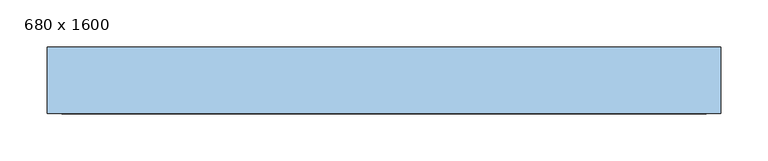
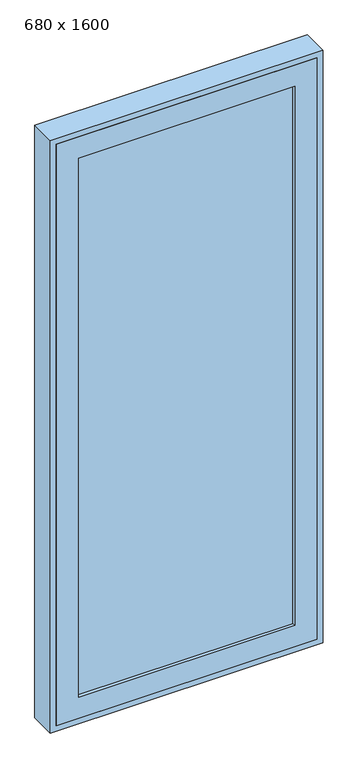
"""IFC4 building model written with IfcOpenShell, lengths in millimetres: window geometry, Aluprof_MB-79N-SI_E_Alu_Window-1sash-FIX_ENG_R-00206 : 680 x 1600."""

from ifc_helpers import new_model, si_unit, frame, origin, place, context, project, spatial, polyline, outline, extrude, faceted_brep, source, transform, mapped, element, save


def window_680_x_1600_1ad14e31(model_context):
    return source(origin(), model_context, "Body", "SolidModel", [
        faceted_brep([(-284.5, -58.5, 2315.5), (-284.5, -58.5, 826.5), (-284.5, -45.0, 826.5), (-284.5, -45.0, 2315.5), (-340.0, -45.0, 2371.0), (-340.0, -45.0, 771.0), (-340.0, -115.0, 771.0), (-340.0, -115.0, 2371.0), (284.5, -58.5, 826.5), (284.5, -45.0, 826.5), (340.0, -45.0, 771.0), (340.0, -115.0, 771.0), (284.5, -58.5, 2315.5), (284.5, -45.0, 2315.5), (340.0, -45.0, 2371.0), (340.0, -115.0, 2371.0), (-300.5, -58.5, 2331.5), (-300.5, -58.5, 810.5), (300.5, -58.5, 810.5), (300.5, -58.5, 2331.5), (-300.5, -106.5, 2331.5), (-300.5, -106.5, 810.5), (300.5, -106.5, 810.5), (300.5, -106.5, 2331.5), (-281.5, -106.5, 2312.5), (-281.5, -106.5, 829.5), (281.5, -106.5, 829.5), (281.5, -106.5, 2312.5), (-281.5, -115.0, 2312.5), (-281.5, -115.0, 829.5), (281.5, -115.0, 829.5), (281.5, -115.0, 2312.5)], [[[0, 1, 2, 3]], [[4, 5, 6, 7]], [[1, 8, 9, 2]], [[5, 10, 11, 6]], [[8, 12, 13, 9]], [[10, 14, 15, 11]], [[16, 17, 18, 19], [1, 0, 12, 8]], [[12, 0, 3, 13]], [[5, 4, 14, 10], [3, 2, 9, 13]], [[14, 4, 7, 15]], [[20, 21, 17, 16]], [[21, 22, 18, 17]], [[22, 23, 19, 18]], [[21, 20, 23, 22], [24, 25, 26, 27]], [[23, 20, 16, 19]], [[28, 29, 25, 24]], [[29, 30, 26, 25]], [[30, 31, 27, 26]], [[7, 6, 11, 15], [29, 28, 31, 30]], [[31, 28, 24, 27]]]),
        extrude(outline(polyline([(300.5, -58.5), (300.5, -106.5), (-300.5, -106.5), (-300.5, -58.5), (300.5, -58.5)])), frame((0.0, 0.0, 810.5), z_axis=(0.0, 0.0, 1.0), x_axis=(1.0, 0.0, 0.0)), (0.0, 0.0, 1.0), 1521.0),
        extrude(outline(polyline([(2386.0, -355.0), (756.0, -355.0), (756.0, 355.0), (2386.0, 355.0), (2386.0, -355.0)]), holes=[polyline([(771.0, -340.0), (2371.0, -340.0), (2371.0, 340.0), (771.0, 340.0), (771.0, -340.0)])]), frame((0.0, -115.0, 0.0), z_axis=(0.0, 1.0, 0.0), x_axis=(0.0, 0.0, 1.0)), (0.0, 0.0, 1.0), 70.0),
    ])


if __name__ == "__main__":
    model = new_model("IFC4")
    model_context = context("Model", 3, world=origin())
    ifc_project = project(units=[si_unit("LENGTHUNIT", "METRE", prefix="MILLI")], contexts=[model_context])
    site = spatial("IfcSite", under=ifc_project)
    building = spatial("IfcBuilding", under=site)
    placement = place(None, origin())
    window_680_x_1600_shape = window_680_x_1600_1ad14e31(model_context)
    element("IfcWindow", 1, ObjectType="Aluprof_MB-79N-SI_E_Alu_Window-1sash-FIX_ENG_R-00206 : 680 x 1600", at=placement, inside=building, context=model_context, shape_type="MappedRepresentation", body=[
        mapped(window_680_x_1600_shape, transform((0.0, 0.0, 0.0), x_axis=(1.0, 0.0, 0.0), y_axis=(0.0, 1.0, 0.0), z_axis=(0.0, 0.0, 1.0))),
    ])
    save(model, "model.ifc")

# Revit data of these elements
# Type "Aluprof_MB-79N-SI_E_Alu_Window-1sash-FIX_ENG_R-00206 : 680 x 1600"
#   Type Mark = "50"
#   Water resistance = "Class E1950, EN 12208"
#   Uniclass2015Version = "v1.6"
#   Uniclass2015Reference = "Pr_30_59_98_02"
#   Uniclass2015Description = "Aluminium window units"
#   URL = "https://aluprof.eu/"
#   Resistance to wind load = "Class C5, EN 12210"
#   Product page URL = "https://aluprof.eu/architekci/katalog-dla-architektow/systemy-okienno-drzwiowe/mb-79n-si-system-okienno-drzwiowy-z-izolacja-termiczna#/materialy/ogolne-informacje"
#   Operation = "SinglePanel"
#   Opening type = "FIX"
#   NBSReference = "45-25-99/310"
#   NBSDescription = "Aluminium window units"
#   Model = "MB-79N SI"
#   Manufacturer = "ALUPROF S.A."
#   Insert type = "SI"
#   IfcExportType = "NOTDEFINED"
#   IfcExportAs = "IfcWindowType"
#   Glazing construction = "6/16/4/16/6"
#   Description = "Single fixed window"
#   Content of the recyclate in the material = "70.7%"
#   COBie.Type.WarrantyDurationParts = ""
#   COBie.Type.Name = ""
#   COBie.Type.Manufacturer = "ALUPROF SA"
#   COBie.Space.Name = ""
#   COBie.Floor.Name = ""
#   COBie.Facility.Name = ""
#   COBie.CreatedOn = ""
#   COBie.CreatedBy = "aluprof.eu"
#   COBie.Component.WarrantyStartDate = ""
#   COBie.Component.Name = "MB-79N SI"
#   Air permeability = "Class 4, EN 12207"
#   Thermal insulation = 0.6000 W/(m²·K)
#   Sash thickness = 79 mm
#   Rough Width = 710 mm
#   Rough Height = 1630 mm
#   Mounting space = 15 mm
#   Height = 1600 mm
#   Glazing area = 0.914121 m²
#   Frame thickness = 70 mm
#   Exterior wall face offset = 60 mm
#   Sill Height = 771 mm
#   Width = 680 mm
#   Warm installation [instance default] = yes
#   Schedule No. [instance default] = 1
#   IsExternal = yes
#   COBie.Type = yes
#   COBie = yes
#   GlazingMaterial = Glass_ALUPROF_Clear
#   FrameMaterial = Träfönster WSP Stockholm
#   BackfillingMaterial = ExpandingFoam_ALUPROF_Yellow
#   Wall Closure = (empty or 0)
# Element 1 (IfcWindow, "Aluprof_MB-79N-SI_E_Alu_Window-1sash-FIX_ENG_R-00206 : 680 x 1600")
#   Materials on its faces: "Träfönster WSP Stockholm", "ExpandingFoam_ALUPROF_Yellow", "Glass_ALUPROF_Clear"
# Materials
#   "Glass_ALUPROF_Clear": class "Glass", colour RGB 22 81 169, transparency 0.85, Model = "GlazingClear", Manufacturer = "ALUPROF S.A.", URL = "https://aluprof.eu/pl-en", Description = "Glazing", Cost = 0
#   "Träfönster WSP Stockholm": class "Generic", colour RGB 45 25 19, transparency 0, Cost = 0
#   "ExpandingFoam_ALUPROF_Yellow": class "Generic", colour RGB 175 175 60, transparency 0, Model = "ExpandingFoam", Manufacturer = "ALUPROF S.A.", URL = "https://aluprof.eu/pl-en", Description = "Expanding foam", Cost = 0
